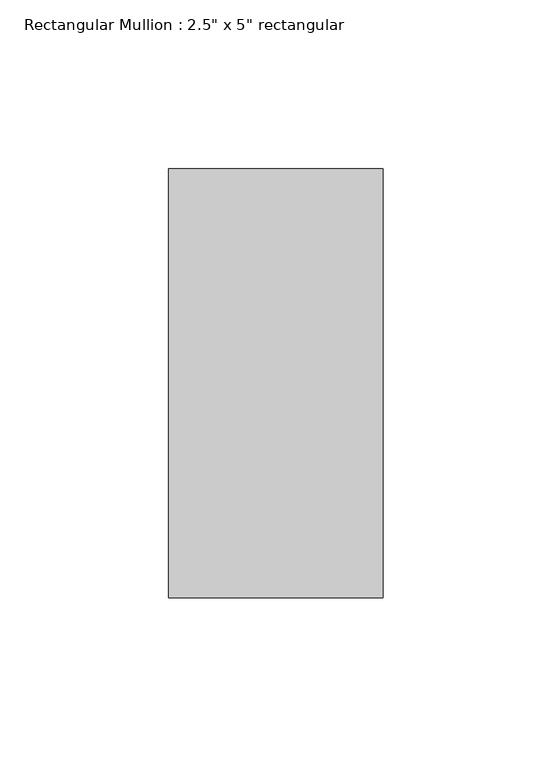
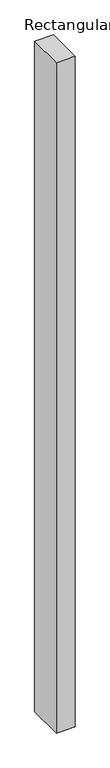
"""IFC4 building model written with IfcOpenShell, lengths in millimetres: member geometry."""

from ifc_helpers import new_model, si_unit, frame, origin, place, context, project, spatial, polyline, outline, extrude, source, transform, mapped, element, save


def member_5511fbbe(model_context):
    return source(origin(), model_context, "Body", "SweptSolid", [
        extrude(outline(polyline([(0.0, 63.5), (0.0, -63.5), (-63.5, -63.5), (-63.5, 63.5), (0.0, 63.5)])), frame((0.0, 0.0, -2398.3630718), z_axis=(0.0, 0.0, 1.0), x_axis=(1.0, 0.0, 0.0)), (0.0, 0.0, 1.0), 2398.3630718),
    ])


if __name__ == "__main__":
    model = new_model("IFC4")
    model_context = context("Model", 3, world=origin())
    ifc_project = project(units=[si_unit("LENGTHUNIT", "METRE", prefix="MILLI")], contexts=[model_context])
    site = spatial("IfcSite", under=ifc_project)
    building = spatial("IfcBuilding", under=site)
    placement = place(None, origin())
    member_shape = member_5511fbbe(model_context)
    element("IfcMember", 1, ObjectType="Rectangular Mullion : 2.5\" x 5\" rectangular", at=placement, inside=building, context=model_context, shape_type="MappedRepresentation", body=[
        mapped(member_shape, transform((0.0, 0.0, 0.0), x_axis=(1.0, 0.0, 0.0), y_axis=(0.0, 1.0, 0.0), z_axis=(0.0, 0.0, 1.0))),
    ])
    save(model, "model.ifc")

# Revit data of these elements
# Type "Rectangular Mullion : 2.5\" x 5\" rectangular"
#   built-in parameter 1007304 = 0.416667 (stored number, unit not read)
#   built-in parameter 1007301 = 0.104167 (stored number, unit not read)
#   built-in parameter 1007300 = 0.104167 (stored number, unit not read)
# Element 1 (IfcMember, "Rectangular Mullion : 2.5\" x 5\" rectangular")
#   Materials on its faces: "Aluminum"
# Materials
#   "Aluminum": class "Metal", colour RGB 247 247 247, transparency 0, Description = "Aluminum 6061", Cost = 0
